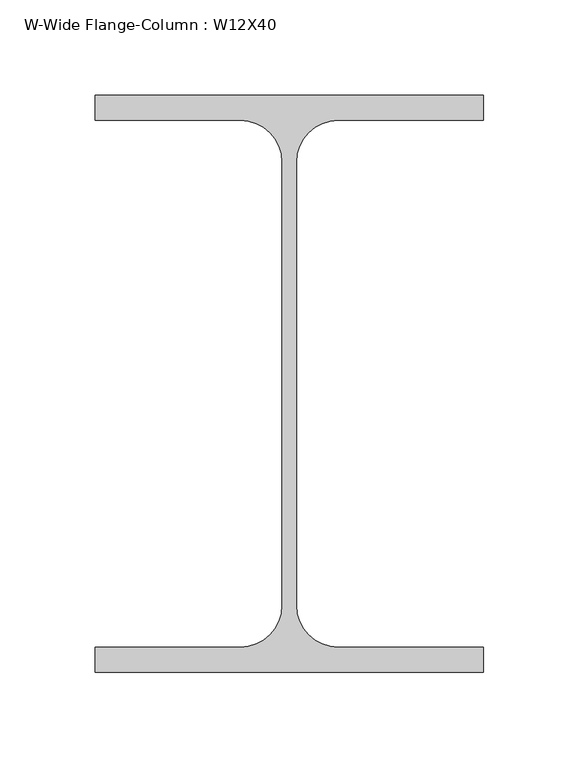
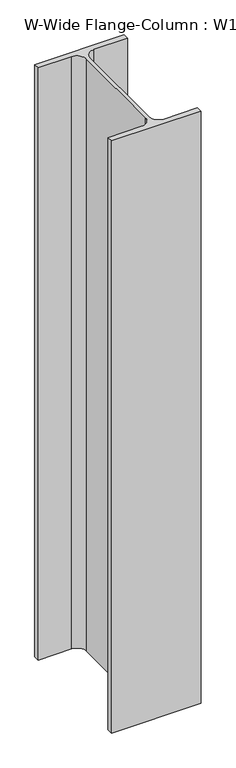
"""IFC4 building model written with IfcOpenShell, lengths in millimetres: column geometry, W-Wide Flange-Column : W12X40."""

from ifc_helpers import new_model, si_unit, point, frame, frame_2d, origin, place, context, project, spatial, polyline, circle_curve, trimmed, segment, composite_curve, outline, extrude, source, transform, mapped, element, save


def w_wide_flange_column_w12x40_5543d8f0(model_context):
    return source(origin(), model_context, "Body", "SweptSolid", [
        extrude(outline(composite_curve([segment(polyline([(101.727, 151.13), (101.727, 138.049), (25.5905, 138.049)]), True, "CONTINUOUS"), segment(trimmed(circle_curve(frame_2d((25.5905, 116.205)), 21.844), [point((25.5905, 138.049))], [point((3.7465, 116.205))], True, "CARTESIAN"), True, "CONTINUOUS"), segment(polyline([(3.7465, 116.205), (3.7465, -116.205)]), True, "CONTINUOUS"), segment(trimmed(circle_curve(frame_2d((25.5905, -116.205)), 21.844), [point((3.7465, -116.205))], [point((25.5905, -138.049))], True, "CARTESIAN"), True, "CONTINUOUS"), segment(polyline([(25.5905, -138.049), (101.727, -138.049), (101.727, -151.13), (-101.727, -151.13), (-101.727, -138.049), (-25.5905, -138.049)]), True, "CONTINUOUS"), segment(trimmed(circle_curve(frame_2d((-25.5905, -116.205)), 21.844), [point((-25.5905, -138.049))], [point((-3.7465, -116.205))], True, "CARTESIAN"), True, "CONTINUOUS"), segment(polyline([(-3.7465, -116.205), (-3.7465, 116.205)]), True, "CONTINUOUS"), segment(trimmed(circle_curve(frame_2d((-25.5905, 116.205)), 21.844), [point((-3.7465, 116.205))], [point((-25.5905, 138.049))], True, "CARTESIAN"), True, "CONTINUOUS"), segment(polyline([(-25.5905, 138.049), (-101.727, 138.049), (-101.727, 151.13), (101.727, 151.13)]), True, "CONTINUOUS")], self_intersect=False)), frame((0.0, 0.0, 17627.6), z_axis=(0.0, 0.0, 1.0), x_axis=(1.0, 0.0, 0.0)), (0.0, 0.0, 1.0), 1422.4),
    ])


if __name__ == "__main__":
    model = new_model("IFC4")
    model_context = context("Model", 3, world=origin())
    ifc_project = project(units=[si_unit("LENGTHUNIT", "METRE", prefix="MILLI")], contexts=[model_context])
    site = spatial("IfcSite", under=ifc_project)
    building = spatial("IfcBuilding", under=site)
    placement = place(None, origin())
    w_wide_flange_column_w12x40_shape = w_wide_flange_column_w12x40_5543d8f0(model_context)
    element("IfcColumn", 1, ObjectType="W-Wide Flange-Column : W12X40", at=placement, inside=building, context=model_context, shape_type="MappedRepresentation", body=[
        mapped(w_wide_flange_column_w12x40_shape, transform((0.0, 0.0, 0.0), x_axis=(1.0, 0.0, 0.0), y_axis=(0.0, 1.0, 0.0), z_axis=(0.0, 0.0, 1.0))),
    ])
    save(model, "model.ifc")

# Revit data of these elements
# Type "W-Wide Flange-Column : W12X40"
#   Assembly Code = "B10"
#   W = 40
#   bf = 0' - 8.01"
#   d = 0' - 11.9"
#   k = 0' - 1 3/8"
#   kr = 0' - 0.86"
#   tf = 0' - 0.515"
#   tw = 0' - 0.295"
#   A = 0.08125 SF
#   Structural Material [instance default] = Steel ASTM A992
# Element 1 (IfcColumn, "W-Wide Flange-Column : W12X40")
#   Materials on its faces: "Steel ASTM A992"
# Materials
#   "Steel ASTM A992": class "Metal", colour RGB 199 199 199, transparency 0, Description = "Structural steel 50ksi", Cost = 0
